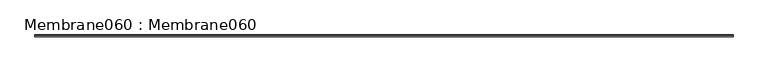
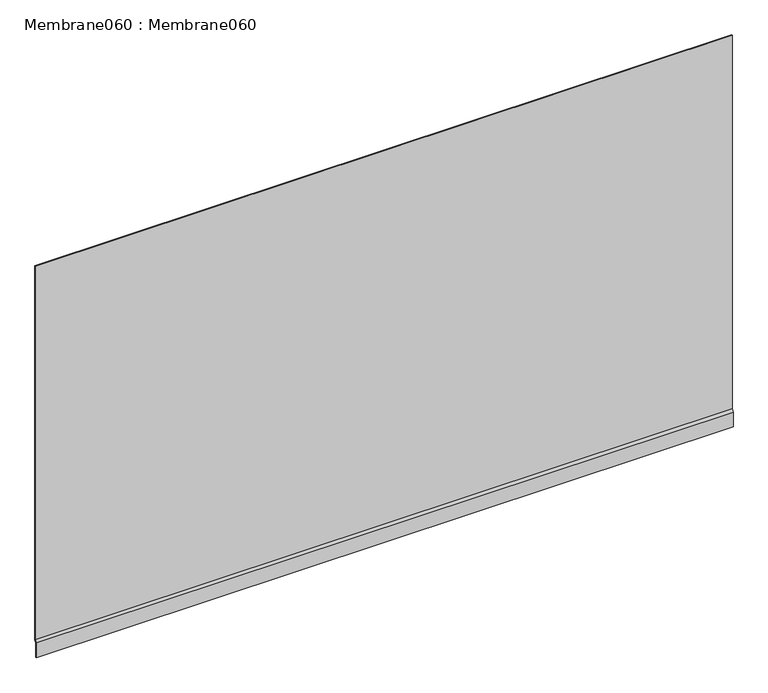
"""IFC4 building model written with IfcOpenShell, lengths in millimetres: proxy geometry, Membrane060 : Membrane060."""

from ifc_helpers import new_model, si_unit, frame, origin, place, context, project, spatial, polyline, outline, extrude, source, transform, mapped, element, save


def membrane060_membrane060_d6b74867(model_context):
    return source(origin(), model_context, "Body", "SweptSolid", [
        extrude(outline(polyline([(4444.6732839, 41689.9549401), (4448.832995, 41696.9627526), (4448.832995, 42830.3967428), (4450.332995, 42830.3967428), (4450.332995, 41696.5510958), (4446.1732839, 41689.5432833), (4446.1732839, 41644.8635958), (4444.6732839, 41644.8635958), (4444.6732839, 41689.9549401)])), frame((255.0171875, 0.0, 0.0), z_axis=(1.0, 0.0, 0.0), x_axis=(0.0, 1.0, 0.0)), (0.0, 0.0, 1.0), 1999.85),
    ])


if __name__ == "__main__":
    model = new_model("IFC4")
    model_context = context("Model", 3, world=origin())
    ifc_project = project(units=[si_unit("LENGTHUNIT", "METRE", prefix="MILLI")], contexts=[model_context])
    site = spatial("IfcSite", under=ifc_project)
    building = spatial("IfcBuilding", under=site)
    placement = place(None, origin())
    membrane060_membrane060_shape = membrane060_membrane060_d6b74867(model_context)
    element("IfcBuildingElementProxy", 1, Name="Membrane060 : Membrane060", ObjectType="Membrane060 : Membrane060", at=placement, inside=building, context=model_context, shape_type="MappedRepresentation", body=[
        mapped(membrane060_membrane060_shape, transform((0.0, 0.0, 0.0), x_axis=(1.0, 0.0, 0.0), y_axis=(0.0, 1.0, 0.0), z_axis=(0.0, 0.0, 1.0))),
    ])
    save(model, "model.ifc")

# Revit data of these elements
# Type "Membrane060 : Membrane060"
#   NameOverride = "Membrane060"
# Element 1 (IfcBuildingElementProxy, "Membrane060 : Membrane060")
#   Materials on its faces: "(2) LAYERS OF ICE & WATER SHIELD (BITUTHANE) UNDER STUCCO"
# Materials
#   "(2) LAYERS OF ICE & WATER SHIELD (BITUTHANE) UNDER STUCCO": class "Unassigned", colour RGB 186 255 159, transparency 0, Cost = 0
